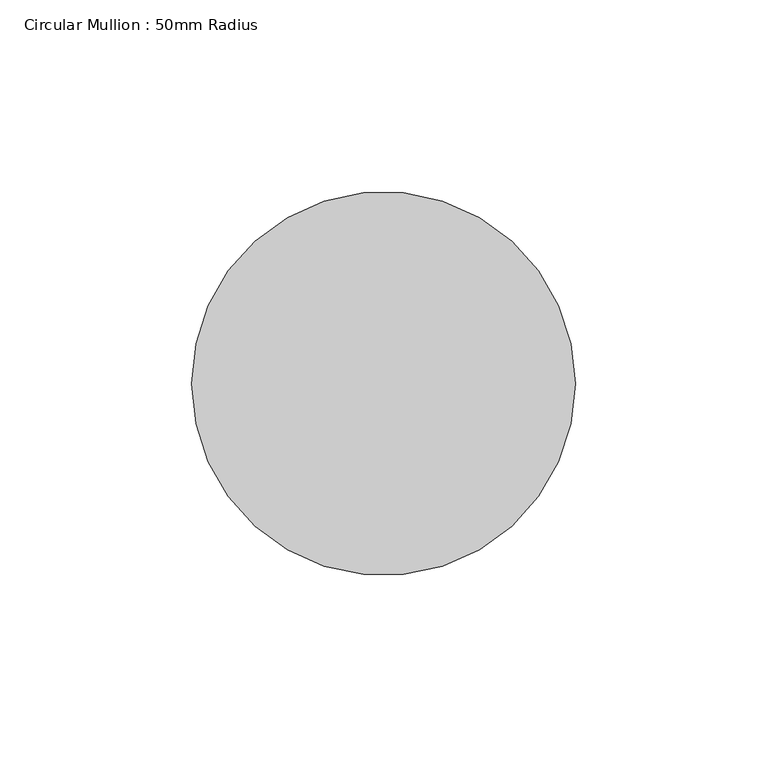
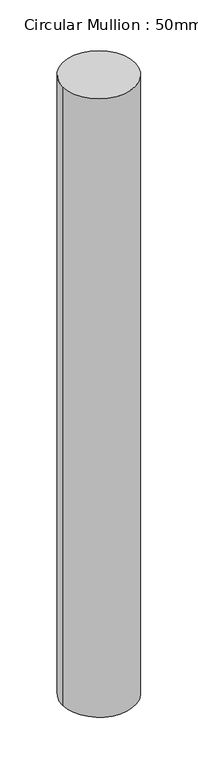
"""IFC4 building model written with IfcOpenShell, lengths in millimetres: member geometry, Circular Mullion : 50mm Radius."""

from ifc_helpers import new_model, si_unit, point, frame, origin, origin_2d, place, context, project, spatial, circle_curve, trimmed, segment, composite_curve, outline, extrude, source, transform, mapped, element, save


def circular_mullion_50mm_radius_e4c24667(model_context):
    return source(origin(), model_context, "Body", "SweptSolid", [
        extrude(outline(composite_curve([segment(trimmed(circle_curve(origin_2d(), 50.0), [point((50.0, 0.0))], [point((-50.0, 0.0))], False, "CARTESIAN"), True, "CONTINUOUS"), segment(trimmed(circle_curve(origin_2d(), 50.0), [point((-50.0, 0.0))], [point((50.0, 0.0))], False, "CARTESIAN"), True, "CONTINUOUS")], self_intersect=False)), frame((0.0, 0.0, -901.3865655), z_axis=(0.0, 0.0, 1.0), x_axis=(1.0, 0.0, 0.0)), (0.0, 0.0, 1.0), 901.3865655),
    ])


if __name__ == "__main__":
    model = new_model("IFC4")
    model_context = context("Model", 3, world=origin())
    ifc_project = project(units=[si_unit("LENGTHUNIT", "METRE", prefix="MILLI")], contexts=[model_context])
    site = spatial("IfcSite", under=ifc_project)
    building = spatial("IfcBuilding", under=site)
    placement = place(None, origin())
    circular_mullion_50mm_radius_shape = circular_mullion_50mm_radius_e4c24667(model_context)
    element("IfcMember", 1, ObjectType="Circular Mullion : 50mm Radius", at=placement, inside=building, context=model_context, shape_type="MappedRepresentation", body=[
        mapped(circular_mullion_50mm_radius_shape, transform((0.0, 0.0, 0.0), x_axis=(1.0, 0.0, 0.0), y_axis=(0.0, 1.0, 0.0), z_axis=(0.0, 0.0, 1.0))),
    ])
    save(model, "model.ifc")

# Revit data of these elements
# Type "Circular Mullion : 50mm Radius"
#   built-in parameter 1007350 = 0.164042 (stored number, unit not read)
# Element 1 (IfcMember, "Circular Mullion : 50mm Radius")
#   Materials on its faces: "Aluminium"
# Materials
#   "Aluminium": class "Metal", colour RGB 247 247 247, transparency 0, Description = "Aluminium 6061", Cost = 0
